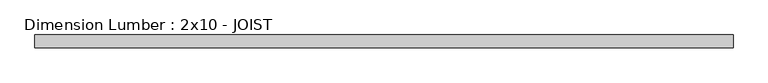
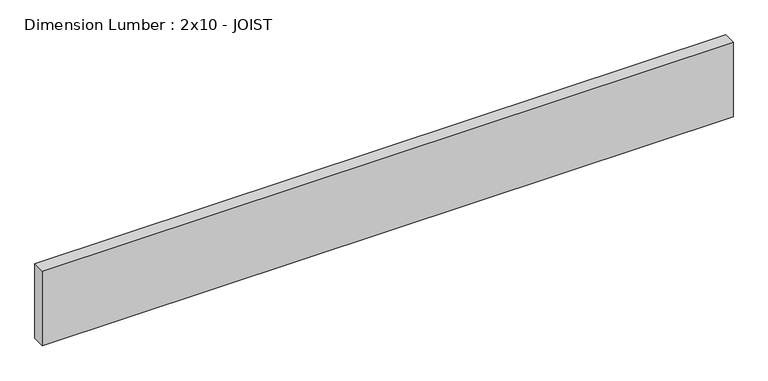
"""IFC4 building model written with IfcOpenShell, lengths in millimetres: beam geometry, Dimension Lumber : 2x10 - JOIST."""

from ifc_helpers import new_model, si_unit, frame, origin, place, context, project, spatial, polyline, outline, extrude, source, transform, mapped, element, save


def dimension_lumber_2x10_joist_4a39c2c6(model_context):
    return source(origin(), model_context, "Body", "SweptSolid", [
        extrude(outline(polyline([(1028.6999994, 19.05), (1028.6999994, -19.05), (-1028.6999994, -19.05), (-1028.6999994, 19.05), (1028.6999994, 19.05)])), frame((0.0, 0.0, -117.475), z_axis=(0.0, 0.0, 1.0), x_axis=(1.0, 0.0, 0.0)), (0.0, 0.0, 1.0), 234.95),
    ])


if __name__ == "__main__":
    model = new_model("IFC4")
    model_context = context("Model", 3, world=origin())
    ifc_project = project(units=[si_unit("LENGTHUNIT", "METRE", prefix="MILLI")], contexts=[model_context])
    site = spatial("IfcSite", under=ifc_project)
    building = spatial("IfcBuilding", under=site)
    placement = place(None, origin())
    dimension_lumber_2x10_joist_shape = dimension_lumber_2x10_joist_4a39c2c6(model_context)
    element("IfcBeam", 1, ObjectType="Dimension Lumber : 2x10 - JOIST", at=placement, inside=building, context=model_context, shape_type="MappedRepresentation", body=[
        mapped(dimension_lumber_2x10_joist_shape, transform((0.0, 0.0, 0.0), x_axis=(1.0, 0.0, 0.0), y_axis=(0.0, 1.0, 0.0), z_axis=(0.0, 0.0, 1.0))),
    ])
    save(model, "model.ifc")

# Revit data of these elements
# Type "Dimension Lumber : 2x10 - JOIST"
#   Assembly Code = "B10"
#   A = 0.0963889 SF
#   Length [instance default] = 5' - 0"
#   b = 0' - 1 1/2"
#   d = 0' - 9 1/4"
#   Structural Material = 2X10 JOISTS
# Element 1 (IfcBeam, "Dimension Lumber : 2x10 - JOIST")
#   Materials on its faces: "2X10 JOISTS"
# Materials
#   "2X10 JOISTS": class "Wood", colour RGB 234 198 147, transparency 0, Description = "Pinus Echinata", Cost = 0
